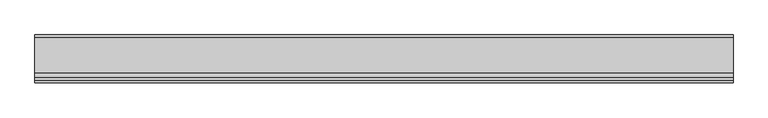
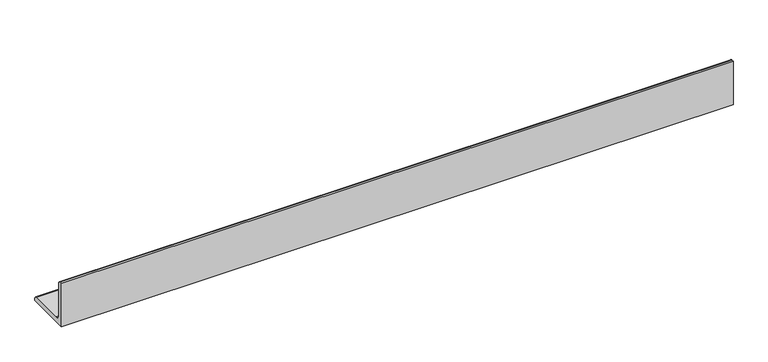
"""IFC4 building model written with IfcOpenShell, lengths in millimetres: beam geometry, NLRS_28_SF_LIB_stalen ligger hoekprofiel gelijkzijdig-AV-MMBS-SRP_gen_rsf : stalen ligger gelijkzijdig hoekprofiel LEQU_gen__150x150x15."""

from ifc_helpers import new_model, si_unit, point, frame, frame_2d, origin, place, context, project, spatial, polyline, circle_curve, trimmed, segment, composite_curve, outline, extrude, source, transform, mapped, element, save


def beam_86464b0d(model_context):
    return source(origin(), model_context, "Body", "SweptSolid", [
        extrude(outline(composite_curve([segment(polyline([(-42.5, -42.5), (-42.5, 107.5), (-35.5, 107.5)]), True, "CONTINUOUS"), segment(trimmed(circle_curve(frame_2d((-35.5, 99.5)), 8.0), [point((-35.5, 107.5))], [point((-27.5, 99.5))], False, "CARTESIAN"), True, "CONTINUOUS"), segment(polyline([(-27.5, 99.5), (-27.5, -11.5)]), True, "CONTINUOUS"), segment(trimmed(circle_curve(frame_2d((-11.5, -11.5)), 16.0), [point((-27.5, -11.5))], [point((-11.5, -27.5))], True, "CARTESIAN"), True, "CONTINUOUS"), segment(polyline([(-11.5, -27.5), (99.5, -27.5)]), True, "CONTINUOUS"), segment(trimmed(circle_curve(frame_2d((99.5, -35.5)), 8.0), [point((99.5, -27.5))], [point((107.5, -35.5))], False, "CARTESIAN"), True, "CONTINUOUS"), segment(polyline([(107.5, -35.5), (107.5, -42.5), (-42.5, -42.5)]), True, "CONTINUOUS")], self_intersect=False)), frame((-1095.0, 0.0, 0.0), z_axis=(1.0, 0.0, 0.0), x_axis=(0.0, 1.0, 0.0)), (0.0, 0.0, 1.0), 2190.0),
    ])


if __name__ == "__main__":
    model = new_model("IFC4")
    model_context = context("Model", 3, world=origin())
    ifc_project = project(units=[si_unit("LENGTHUNIT", "METRE", prefix="MILLI")], contexts=[model_context])
    site = spatial("IfcSite", under=ifc_project)
    building = spatial("IfcBuilding", under=site)
    placement = place(None, origin())
    beam_shape = beam_86464b0d(model_context)
    element("IfcBeam", 1, ObjectType="NLRS_28_SF_LIB_stalen ligger hoekprofiel gelijkzijdig-AV-MMBS-SRP_gen_rsf : stalen ligger gelijkzijdig hoekprofiel LEQU_gen__150x150x15", at=placement, inside=building, context=model_context, shape_type="MappedRepresentation", body=[
        mapped(beam_shape, transform((0.0, 0.0, 0.0), x_axis=(1.0, 0.0, 0.0), y_axis=(0.0, 1.0, 0.0), z_axis=(0.0, 0.0, 1.0))),
    ])
    save(model, "model.ifc")

# Revit data of these elements
# Type "NLRS_28_SF_LIB_stalen ligger hoekprofiel gelijkzijdig-AV-MMBS-SRP_gen_rsf : stalen ligger gelijkzijdig hoekprofiel LEQU_gen__150x150x15"
#   Type IfcGUID = "2CEqVLPNH8KRN7ghwV3a1U"
#   IfcExportAs = "IfcBeamType"
#   Type Comments = "L150x150x15"
#   Model = " "
#   Manufacturer = " "
#   Fire Rating = " "
#   Description = "stalen ligger L150x150x15"
#   Assembly Code = "28.11"
#   vz = 107.5 mm
#   vy = 107.5 mm
#   tw = 15 mm
#   tf = 15 mm
#   ri = 8 mm
#   ra = 16 mm
#   d = 150 mm
#   bf = 150 mm
#   NLRS_C_lengte [instance default] = 1524 mm
#   Length [instance default] = 1524 mm
#   Structural Material = NLRS_h2_staal_gen_rsf
#   Keynote = ""
# Element 1 (IfcBeam, "NLRS_28_SF_LIB_stalen ligger hoekprofiel gelijkzijdig-AV-MMBS-SRP_gen_rsf : stalen ligger gelijkzijdig hoekprofiel LEQU_gen__150x150x15")
#   NLRS_C_lengte = 2190 mm
#   Materials on its faces: "NLRS_h2_staal_gen_rsf"
# Materials
#   "NLRS_h2_staal_gen_rsf": class "H - Metaal", colour RGB 189 187 185, transparency 0, Keynote = "h2", Manufacturer = "Revit Standards Foundation", URL = "www.revitstandards.org", Description = "staal", Cost = 0
